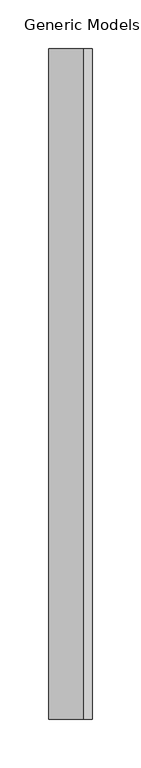
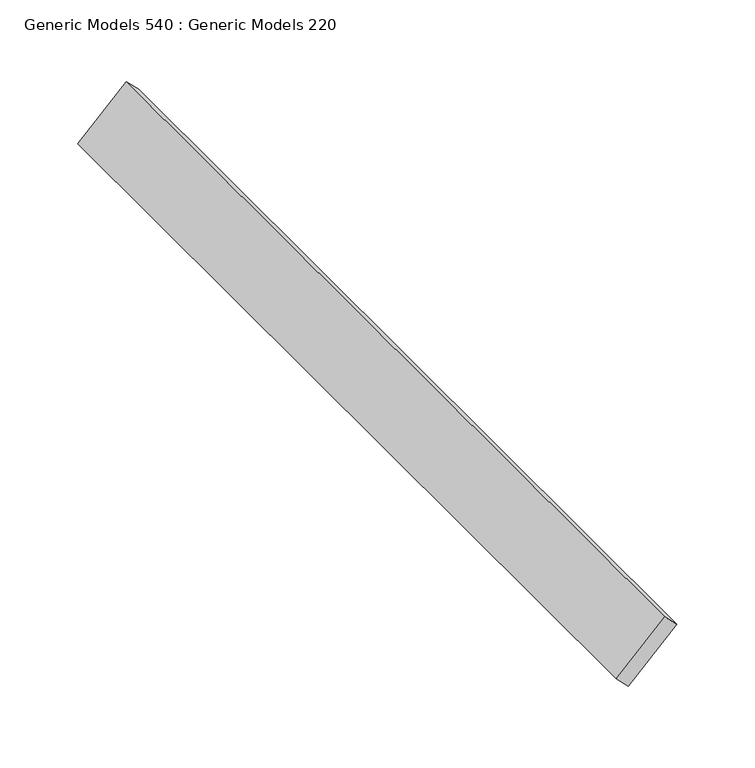
"""IFC4 building model written with IfcOpenShell, lengths in millimetres: proxy geometry, Generic Models 540 : Generic Models 220."""

from ifc_helpers import new_model, si_unit, frame, origin, place, context, project, spatial, polyline, outline, extrude, source, transform, mapped, element, save


def generic_models_540_generic_models_220_b31f382a(model_context):
    return source(origin(), model_context, "Body", "SweptSolid", [
        extrude(outline(polyline([(0.0, -12.7000001), (0.0, 0.0), (690.8142348, 0.0), (690.8142348, -12.7000001), (0.0, -12.7000001)])), frame((7841.3059863, 4539.4872686, 125001.6399101), z_axis=(0.7071067811868034, 0.0, 0.7071067811862918), x_axis=(0.0, -1.0, 0.0)), (0.0, 0.0, 1.0), 50.8),
    ])


if __name__ == "__main__":
    model = new_model("IFC4")
    model_context = context("Model", 3, world=origin())
    ifc_project = project(units=[si_unit("LENGTHUNIT", "METRE", prefix="MILLI")], contexts=[model_context])
    site = spatial("IfcSite", under=ifc_project)
    building = spatial("IfcBuilding", under=site)
    placement = place(None, origin())
    generic_models_540_generic_models_220_shape = generic_models_540_generic_models_220_b31f382a(model_context)
    element("IfcBuildingElementProxy", 1, Name="Generic Models 540 : Generic Models 220", ObjectType="Generic Models 540 : Generic Models 220", at=placement, inside=building, context=model_context, shape_type="MappedRepresentation", body=[
        mapped(generic_models_540_generic_models_220_shape, transform((0.0, 0.0, 0.0), x_axis=(1.0, 0.0, 0.0), y_axis=(0.0, 1.0, 0.0), z_axis=(0.0, 0.0, 1.0))),
    ])
    save(model, "model.ifc")

# Revit data of these elements
# Element 1 (IfcBuildingElementProxy, "Generic Models 540 : Generic Models 220")
#   Materials on its faces: "_WOOD TONE ALUMINUM EXTRUSION SLAT BY KNOTWOOD"
# Materials
#   "_WOOD TONE ALUMINUM EXTRUSION SLAT BY KNOTWOOD": class "Generic", colour RGB 177 130 114, transparency 0, Cost = 0
